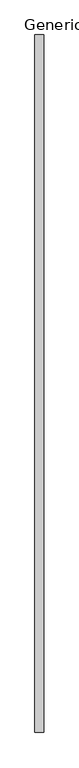
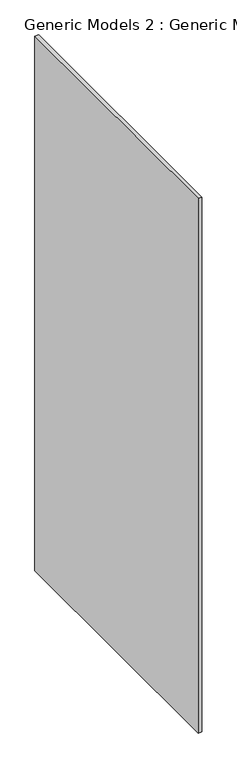
"""IFC4 building model written with IfcOpenShell, lengths in millimetres: proxy geometry, Generic Models 2 : Generic Models 1."""

from ifc_helpers import new_model, si_unit, frame, origin, place, context, project, spatial, polyline, outline, extrude, source, transform, mapped, element, save


def generic_models_2_generic_models_1_35b0c06a(model_context):
    return source(origin(), model_context, "Body", "SweptSolid", [
        extrude(outline(polyline([(49799.875, 1219.2), (49799.875, 0.0), (49784.0, 0.0), (49784.0, 1219.2), (49799.875, 1219.2)])), frame((0.0, 0.0, 3054.35), z_axis=(0.0, 0.0, 1.0), x_axis=(1.0, 0.0, 0.0)), (0.0, 0.0, 1.0), 2438.4),
    ])


if __name__ == "__main__":
    model = new_model("IFC4")
    model_context = context("Model", 3, world=origin())
    ifc_project = project(units=[si_unit("LENGTHUNIT", "METRE", prefix="MILLI")], contexts=[model_context])
    site = spatial("IfcSite", under=ifc_project)
    building = spatial("IfcBuilding", under=site)
    placement = place(None, origin())
    generic_models_2_generic_models_1_shape = generic_models_2_generic_models_1_35b0c06a(model_context)
    element("IfcBuildingElementProxy", 1, Name="Generic Models 2 : Generic Models 1", ObjectType="Generic Models 2 : Generic Models 1", at=placement, inside=building, context=model_context, shape_type="MappedRepresentation", body=[
        mapped(generic_models_2_generic_models_1_shape, transform((0.0, 0.0, 0.0), x_axis=(1.0, 0.0, 0.0), y_axis=(0.0, 1.0, 0.0), z_axis=(0.0, 0.0, 1.0))),
    ])
    save(model, "model.ifc")

# Revit data of these elements
# Element 1 (IfcBuildingElementProxy, "Generic Models 2 : Generic Models 1")
#   Materials on its faces: "GYP. BD (SEE 'WALL TAG' & 'LAYER MATERIAL SCHEDULE' FOR DETAILS)"
# Materials
#   "GYP. BD (SEE 'WALL TAG' & 'LAYER MATERIAL SCHEDULE' FOR DETAILS)": class "Generic", colour RGB 237 236 233, transparency 0, Description = "Gypsum Wall Board", Cost = 0
